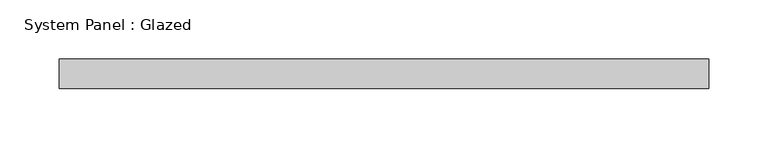
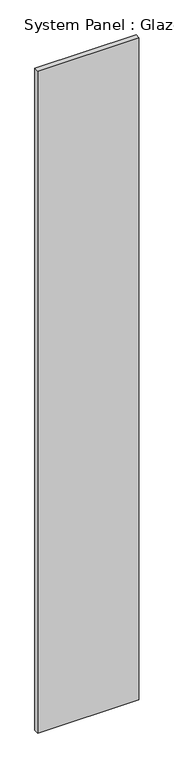
"""IFC4 building model written with IfcOpenShell, lengths in millimetres: plate geometry, System Panel : Glazed."""

from ifc_helpers import new_model, si_unit, origin, origin_with_axes, place, context, project, spatial, polyline, outline, extrude, source, transform, mapped, element, save


def system_panel_glazed_e3bcbcf3(model_context):
    return source(origin(), model_context, "Body", "SweptSolid", [
        extrude(outline(polyline([(274.9999998, 24.5), (-274.9999998, 24.5), (-274.9999998, 49.5), (274.9999998, 49.5), (274.9999998, 24.5)])), origin_with_axes(), (0.0, 0.0, 1.0), 3800.0),
    ])


if __name__ == "__main__":
    model = new_model("IFC4")
    model_context = context("Model", 3, world=origin())
    ifc_project = project(units=[si_unit("LENGTHUNIT", "METRE", prefix="MILLI")], contexts=[model_context])
    site = spatial("IfcSite", under=ifc_project)
    building = spatial("IfcBuilding", under=site)
    placement = place(None, origin())
    system_panel_glazed_shape = system_panel_glazed_e3bcbcf3(model_context)
    element("IfcPlate", 1, ObjectType="System Panel : Glazed", at=placement, inside=building, context=model_context, shape_type="MappedRepresentation", body=[
        mapped(system_panel_glazed_shape, transform((0.0, 0.0, 0.0), x_axis=(1.0, 0.0, 0.0), y_axis=(0.0, 1.0, 0.0), z_axis=(0.0, 0.0, 1.0))),
    ])
    save(model, "model.ifc")

# Revit data of these elements
# Type "System Panel : Glazed"
#   Construction Type Id = "GSP4R"
#   Analytic Construction = "1/8 in Pilkington single glazing"
#   Visual Light Transmittance = 0.9
#   Solar Heat Gain Coefficient = 0.86
#   Heat Transfer Coefficient (U) = 6.7069 W/(m²·K)
#   Define Thermal Properties by = 1
# Element 1 (IfcPlate, "System Panel : Glazed")
#   Materials on its faces: "Glass"
# Materials
#   "Glass": class "Glass", colour RGB 0 128 192, transparency 0.9, Description = "Soda Lime Glass", Cost = 0
